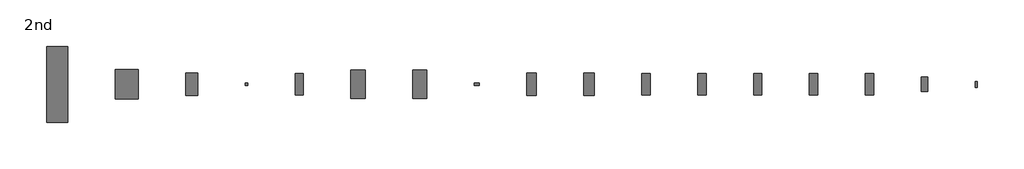
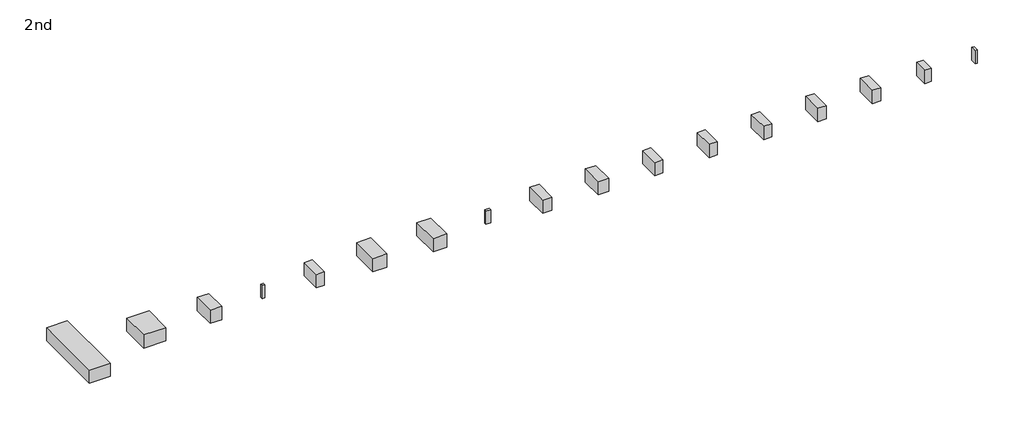
# One storey: 17 proxies.
"""IFC4 building model written with IfcOpenShell, lengths in millimetres."""

import ifcopenshell
import ifcopenshell.guid

model = None  # the IFC model being written
_history = None  # IfcOwnerHistory: only IFC2X3 demands one
_inside = {}  # id of a spatial element -> (the spatial element, [elements in it])
_under = {}  # id of a project, library or spatial element -> (it, [spatial elements below it])
_declared = {}  # id of a project -> (the project, [libraries it declares])
_typed = {}  # id of a type object -> (the type object, [elements of that type])
_made_of = {}  # id of a material, layer set ... -> (it, [elements and type objects made of it])


def new_model(schema):
    """Start an empty IFC model of exactly this schema.

    Asked for "IFC4X3", IfcOpenShell would pick the latest addendum, in which some entities
    have other attributes; the version numbers below select the first issue.
    IFC2X3 requires an IfcOwnerHistory on every rooted entity: one is made here for all.
    """
    global model, _history
    if schema == "IFC4X3":
        model = ifcopenshell.file(schema_version=(4, 3, 0, 0))
    else:
        model = ifcopenshell.file(schema=schema)
    _inside.clear()
    _under.clear()
    _declared.clear()
    _typed.clear()
    _made_of.clear()
    _history = None
    if model.schema == "IFC2X3":
        org = make("IfcOrganization", Name="unknown")
        user = make(
            "IfcPersonAndOrganization",
            ThePerson=make("IfcPerson", FamilyName="unknown"),
            TheOrganization=org,
        )
        app = make(
            "IfcApplication",
            ApplicationDeveloper=org,
            Version="unknown",
            ApplicationFullName="unknown",
            ApplicationIdentifier="unknown",
        )
        _history = make(
            "IfcOwnerHistory",
            OwningUser=user,
            OwningApplication=app,
            ChangeAction="ADDED",
            CreationDate=0,
        )
    return model


def make(cls, **values):
    """One entity of the class cls with the attributes given. An attribute that is None is left unset."""
    return model.create_entity(
        cls, **{name: value for name, value in values.items() if value is not None}
    )


def rooted(cls, **values):
    """An entity with a GlobalId (a new one), such as an element, a storey or a relation."""
    return make(cls, GlobalId=ifcopenshell.guid.new(), OwnerHistory=_history, **values)


def si_unit(unit_type, name, prefix=None):
    """IfcSIUnit, for example si_unit("LENGTHUNIT", "METRE", prefix="MILLI")."""
    return make("IfcSIUnit", UnitType=unit_type, Prefix=prefix, Name=name)


def assignment(units):
    """IfcUnitAssignment: the units of a project."""
    return None if units is None else make("IfcUnitAssignment", Units=units)


def point(xyz):
    """IfcCartesianPoint."""
    return None if xyz is None else make("IfcCartesianPoint", Coordinates=xyz)


def direction(xyz):
    """IfcDirection."""
    return None if xyz is None else make("IfcDirection", DirectionRatios=xyz)


def frame(location, z_axis=None, x_axis=None):
    """IfcAxis2Placement3D, a coordinate frame: its origin and axes. An axis left out is left unset."""
    return make(
        "IfcAxis2Placement3D",
        Location=point(location),
        Axis=direction(z_axis),
        RefDirection=direction(x_axis),
    )


def origin():
    """The frame at (0, 0, 0) with its axes left unset."""
    return frame((0.0, 0.0, 0.0))


def origin_with_axes():
    """The frame at (0, 0, 0) with the z axis (0, 0, 1) and the x axis (1, 0, 0) written out."""
    return frame((0.0, 0.0, 0.0), z_axis=(0.0, 0.0, 1.0), x_axis=(1.0, 0.0, 0.0))


def place(relative_to, where):
    """IfcLocalPlacement: puts the frame where relative to a parent placement (None: the world)."""
    return make(
        "IfcLocalPlacement", PlacementRelTo=relative_to, RelativePlacement=where
    )


def context(
    kind, dimensions, precision=None, world=None, true_north=None, identifier=None
):
    """IfcGeometricRepresentationContext, for example the 3D "Model" context."""
    return make(
        "IfcGeometricRepresentationContext",
        ContextIdentifier=identifier,
        ContextType=kind,
        CoordinateSpaceDimension=dimensions,
        Precision=precision,
        WorldCoordinateSystem=world,
        TrueNorth=true_north,
    )


def project(units=None, contexts=None):
    """IfcProject with its units and contexts."""
    return rooted(
        "IfcProject",
        Name="project",
        RepresentationContexts=contexts,
        UnitsInContext=assignment(units),
    )


def spatial(cls, under=None, at=None, **own):
    """A site, building, storey or space (cls), placed at a placement, below another one or the project."""
    s = rooted(cls, ObjectPlacement=at, **own)
    if under is not None:
        _under.setdefault(under.id(), (under, []))[1].append(s)
    return s


def polyline(points):
    """IfcPolyline through the points."""
    return make("IfcPolyline", Points=[point(p) for p in points])


def outline(outer, holes=None, kind="AREA"):
    """IfcArbitraryClosedProfileDef: a profile drawn as a closed curve; with holes, ...WithVoids."""
    if holes is None:
        return make("IfcArbitraryClosedProfileDef", ProfileType=kind, OuterCurve=outer)
    return make(
        "IfcArbitraryProfileDefWithVoids",
        ProfileType=kind,
        OuterCurve=outer,
        InnerCurves=holes,
    )


def extrude(swept, where, along, depth):
    """IfcExtrudedAreaSolid: the profile swept, set in the frame where, extruded along a direction by depth."""
    return make(
        "IfcExtrudedAreaSolid",
        SweptArea=swept,
        Position=where,
        ExtrudedDirection=direction(along),
        Depth=depth,
    )


def shape(context_of_items, identifier, shape_type, items):
    """IfcShapeRepresentation: the items that make up one representation, for example the "Body"."""
    return make(
        "IfcShapeRepresentation",
        ContextOfItems=context_of_items,
        RepresentationIdentifier=identifier,
        RepresentationType=shape_type,
        Items=items,
    )


def source(mapping_origin, context_of_items, identifier, shape_type, items):
    """IfcRepresentationMap: a shape defined once, which mapped items show again and again."""
    return make(
        "IfcRepresentationMap",
        MappingOrigin=mapping_origin,
        MappedRepresentation=shape(context_of_items, identifier, shape_type, items),
    )


def transform(
    local_origin,
    x_axis=None,
    y_axis=None,
    z_axis=None,
    scale=None,
    scale2=None,
    scale3=None,
    uniform=True,
):
    """IfcCartesianTransformationOperator3D, or its non-uniform kind. x_axis, y_axis, z_axis: its Axis1, 2, 3."""
    if uniform:
        return make(
            "IfcCartesianTransformationOperator3D",
            Axis1=direction(x_axis),
            Axis2=direction(y_axis),
            LocalOrigin=point(local_origin),
            Scale=scale,
            Axis3=direction(z_axis),
        )
    return make(
        "IfcCartesianTransformationOperator3DnonUniform",
        Axis1=direction(x_axis),
        Axis2=direction(y_axis),
        LocalOrigin=point(local_origin),
        Scale=scale,
        Axis3=direction(z_axis),
        Scale2=scale2,
        Scale3=scale3,
    )


def mapped(mapping_source, mapping_target):
    """IfcMappedItem: shows the shape of a source again, moved by a transform."""
    return make(
        "IfcMappedItem", MappingSource=mapping_source, MappingTarget=mapping_target
    )


def made_of(thing, what):
    """Note that an element or type object is made of a material, layer set ...; save() writes the relation."""
    if what is not None:
        _made_of.setdefault(what.id(), (what, []))[1].append(thing)
    return thing


def element(
    cls,
    number,
    at=None,
    inside=None,
    cuts=None,
    type_object=None,
    material=None,
    context=None,
    identifier="Body",
    shape_type=None,
    held_by="IfcProductDefinitionShape",
    body=None,
    shapes=None,
    **own,
):
    """One element of the class cls, such as IfcWall. Its Tag is "e" and its number.

    at: its placement. inside: the storey or other place that contains it. cuts: it is an
    opening in that element (IfcRelVoidsElement). A single representation is given by context,
    identifier, shape_type and body (its items); several are given by shapes. held_by: the class
    of the entity that holds the representations. save() writes the other relations.
    """
    e = rooted(cls, Tag="e%d" % number, ObjectPlacement=at, **own)
    if body is not None:
        shapes = [shape(context, identifier, shape_type, body)]
    if shapes is not None:
        e.Representation = make(held_by, Representations=shapes)
    if inside is not None:
        _inside.setdefault(inside.id(), (inside, []))[1].append(e)
    if cuts is not None:
        rooted(
            "IfcRelVoidsElement", RelatingBuildingElement=cuts, RelatedOpeningElement=e
        )
    if type_object is not None:
        _typed.setdefault(type_object.id(), (type_object, []))[1].append(e)
    return made_of(e, material)


def aggregate(whole, parts):
    """IfcRelAggregates: a whole, such as a stair, and the parts it consists of."""
    return rooted("IfcRelAggregates", RelatingObject=whole, RelatedObjects=parts)


def save(model, path):
    """Write the relations noted so far, then the file.

    IfcRelAggregates (storeys below a building ...), IfcRelContainedInSpatialStructure (elements
    in a storey), IfcRelDefinesByType, IfcRelAssociatesMaterial and IfcRelDeclares: one each for
    every whole, place, type object, material and project.
    """
    for whole, parts in _under.values():
        aggregate(whole, parts)
    for where, things in _inside.values():
        rooted(
            "IfcRelContainedInSpatialStructure",
            RelatedElements=things,
            RelatingStructure=where,
        )
    for kind, things in _typed.values():
        rooted("IfcRelDefinesByType", RelatedObjects=things, RelatingType=kind)
    for what, things in _made_of.values():
        rooted("IfcRelAssociatesMaterial", RelatedObjects=things, RelatingMaterial=what)
    for by, libraries in _declared.values():
        rooted("IfcRelDeclares", RelatingContext=by, RelatedDefinitions=libraries)
    model.write(path)


def generic_models_5634f436(model_context):
    return source(origin(), model_context, "Body", "SweptSolid", [
        extrude(outline(polyline([(1350.0, 3000.0), (1350.0, -3000.0), (-1350.0, -3000.0), (-1350.0, 3000.0), (1350.0, 3000.0)])), origin_with_axes(), (0.0, 0.0, 1.0), 6000.0),
    ])


def generic_models_71e2440f(model_context):
    return source(origin(), model_context, "Body", "SweptSolid", [
        extrude(outline(polyline([(500.0, 1250.0), (500.0, -1250.0), (-500.0, -1250.0), (-500.0, 1250.0), (500.0, 1250.0)])), origin_with_axes(), (0.0, 0.0, 1.0), 6000.0),
    ])


def generic_models_57c7875f(model_context):
    return source(origin(), model_context, "Body", "SweptSolid", [
        extrude(outline(polyline([(4500.0, 16000.0), (4500.0, -16000.0), (-4500.0, -16000.0), (-4500.0, 16000.0), (4500.0, 16000.0)])), origin_with_axes(), (0.0, 0.0, 1.0), 6000.0),
    ])


def generic_models_72d488a7(model_context):
    return source(origin(), model_context, "Body", "SweptSolid", [
        extrude(outline(polyline([(4800.0, 6250.0), (4800.0, -6250.0), (-4800.0, -6250.0), (-4800.0, 6250.0), (4800.0, 6250.0)])), origin_with_axes(), (0.0, 0.0, 1.0), 6000.0),
    ])


def generic_models_7902148a(model_context):
    return source(origin(), model_context, "Body", "SweptSolid", [
        extrude(outline(polyline([(2500.0, 4800.0), (2500.0, -4800.0), (-2500.0, -4800.0), (-2500.0, 4800.0), (2500.0, 4800.0)])), origin_with_axes(), (0.0, 0.0, 1.0), 6000.0),
    ])


def generic_models_ed4b717c(model_context):
    return source(origin(), model_context, "Body", "SweptSolid", [
        extrude(outline(polyline([(500.0, 500.0), (500.0, -500.0), (-500.0, -500.0), (-500.0, 500.0), (500.0, 500.0)])), origin_with_axes(), (0.0, 0.0, 1.0), 6000.0),
    ])


def generic_models_c01b8d6f(model_context):
    return source(origin(), model_context, "Body", "SweptSolid", [
        extrude(outline(polyline([(1750.0, 4500.0), (1750.0, -4500.0), (-1750.0, -4500.0), (-1750.0, 4500.0), (1750.0, 4500.0)])), origin_with_axes(), (0.0, 0.0, 1.0), 6000.0),
    ])


def generic_models_43059f4e(model_context):
    return source(origin(), model_context, "Body", "SweptSolid", [
        extrude(outline(polyline([(3000.0, 6000.0), (3000.0, -6000.0), (-3000.0, -6000.0), (-3000.0, 6000.0), (3000.0, 6000.0)])), origin_with_axes(), (0.0, 0.0, 1.0), 6000.0),
    ])


def generic_models_da00a96f(model_context):
    return source(origin(), model_context, "Body", "SweptSolid", [
        extrude(outline(polyline([(1000.0, 500.0), (1000.0, -500.0), (-1000.0, -500.0), (-1000.0, 500.0), (1000.0, 500.0)])), origin_with_axes(), (0.0, 0.0, 1.0), 6000.0),
    ])


def generic_models_3a820573(model_context):
    return source(origin(), model_context, "Body", "SweptSolid", [
        extrude(outline(polyline([(2000.0, 4750.0), (2000.0, -4750.0), (-2000.0, -4750.0), (-2000.0, 4750.0), (2000.0, 4750.0)])), origin_with_axes(), (0.0, 0.0, 1.0), 6000.0),
    ])


def generic_models_96097b63(model_context):
    return source(origin(), model_context, "Body", "SweptSolid", [
        extrude(outline(polyline([(2250.0, 4800.0), (2250.0, -4800.0), (-2250.0, -4800.0), (-2250.0, 4800.0), (2250.0, 4800.0)])), origin_with_axes(), (0.0, 0.0, 1.0), 6000.0),
    ])


model = new_model("IFC4")

# Units and contexts
model_context = context("Model", 3, world=origin())
ifc_project = project(units=[si_unit("LENGTHUNIT", "METRE", prefix="MILLI")], contexts=[model_context])

# Site, building, storey
site = spatial("IfcSite", under=ifc_project)
building = spatial("IfcBuilding", under=site)
storey = spatial("IfcBuildingStorey", under=building, Name="2nd", Elevation=14000.0)

# Proxies
placement = place(None, origin())
generic_models_shape = generic_models_5634f436(model_context)
element("IfcBuildingElementProxy", 1, Name="Space Planning Box_hec : Space Planning Box_hec", ObjectType="Space Planning Box_hec : Space Planning Box_hec", at=placement, inside=storey, context=model_context, shape_type="MappedRepresentation", body=[
    mapped(generic_models_shape, transform((369450.0, 168000.0, 14000.0), x_axis=(1.0, 0.0, 0.0), y_axis=(0.0, 1.0, 0.0), z_axis=(0.0, 0.0, 1.0))),
])
generic_models_2_shape = generic_models_71e2440f(model_context)
element("IfcBuildingElementProxy", 2, Name="Space Planning Box_hec : Space Planning Box_hec", ObjectType="Space Planning Box_hec : Space Planning Box_hec", at=placement, inside=storey, context=model_context, shape_type="MappedRepresentation", body=[
    mapped(generic_models_2_shape, transform((391300.0, 168000.0, 14000.0), x_axis=(1.0, 0.0, 0.0), y_axis=(0.0, 1.0, 0.0), z_axis=(0.0, 0.0, 1.0))),
])
generic_models_3_shape = generic_models_57c7875f(model_context)
element("IfcBuildingElementProxy", 3, Name="Space Planning Box_hec : Space Planning Box_hec", ObjectType="Space Planning Box_hec : Space Planning Box_hec", at=placement, inside=storey, context=model_context, shape_type="MappedRepresentation", body=[
    mapped(generic_models_3_shape, transform((4500.0, 168000.0, 14000.0), x_axis=(1.0, 0.0, 0.0), y_axis=(0.0, 1.0, 0.0), z_axis=(0.0, 0.0, 1.0))),
])
generic_models_4_shape = generic_models_72d488a7(model_context)
element("IfcBuildingElementProxy", 4, Name="Space Planning Box_hec : Space Planning Box_hec", ObjectType="Space Planning Box_hec : Space Planning Box_hec", at=placement, inside=storey, context=model_context, shape_type="MappedRepresentation", body=[
    mapped(generic_models_4_shape, transform((33800.0, 168000.0, 14000.0), x_axis=(1.0, 0.0, 0.0), y_axis=(0.0, 1.0, 0.0), z_axis=(0.0, 0.0, 1.0))),
])
generic_models_5_shape = generic_models_7902148a(model_context)
element("IfcBuildingElementProxy", 5, Name="Space Planning Box_hec : Space Planning Box_hec", ObjectType="Space Planning Box_hec : Space Planning Box_hec", at=placement, inside=storey, context=model_context, shape_type="MappedRepresentation", body=[
    mapped(generic_models_5_shape, transform((61100.0, 168000.0, 14000.0), x_axis=(1.0, 0.0, 0.0), y_axis=(0.0, 1.0, 0.0), z_axis=(0.0, 0.0, 1.0))),
])
generic_models_6_shape = generic_models_ed4b717c(model_context)
element("IfcBuildingElementProxy", 6, Name="Space Planning Box_hec : Space Planning Box_hec", ObjectType="Space Planning Box_hec : Space Planning Box_hec", at=placement, inside=storey, context=model_context, shape_type="MappedRepresentation", body=[
    mapped(generic_models_6_shape, transform((84100.0, 168000.0, 14000.0), x_axis=(1.0, 0.0, 0.0), y_axis=(0.0, 1.0, 0.0), z_axis=(0.0, 0.0, 1.0))),
])
generic_models_7_shape = generic_models_c01b8d6f(model_context)
element("IfcBuildingElementProxy", 7, Name="Space Planning Box_hec : Space Planning Box_hec", ObjectType="Space Planning Box_hec : Space Planning Box_hec", at=placement, inside=storey, context=model_context, shape_type="MappedRepresentation", body=[
    mapped(generic_models_7_shape, transform((106350.0, 168000.0, 14000.0), x_axis=(1.0, 0.0, 0.0), y_axis=(0.0, 1.0, 0.0), z_axis=(0.0, 0.0, 1.0))),
])
element("IfcBuildingElementProxy", 8, Name="Space Planning Box_hec : Space Planning Box_hec", ObjectType="Space Planning Box_hec : Space Planning Box_hec", at=placement, inside=storey, context=model_context, shape_type="MappedRepresentation", body=[
    mapped(generic_models_7_shape, transform((252350.0, 168000.0, 14000.0), x_axis=(1.0, 0.0, 0.0), y_axis=(0.0, 1.0, 0.0), z_axis=(0.0, 0.0, 1.0))),
])
element("IfcBuildingElementProxy", 9, Name="Space Planning Box_hec : Space Planning Box_hec", ObjectType="Space Planning Box_hec : Space Planning Box_hec", at=placement, inside=storey, context=model_context, shape_type="MappedRepresentation", body=[
    mapped(generic_models_7_shape, transform((275850.0, 168000.0, 14000.0), x_axis=(1.0, 0.0, 0.0), y_axis=(0.0, 1.0, 0.0), z_axis=(0.0, 0.0, 1.0))),
])
element("IfcBuildingElementProxy", 10, Name="Space Planning Box_hec : Space Planning Box_hec", ObjectType="Space Planning Box_hec : Space Planning Box_hec", at=placement, inside=storey, context=model_context, shape_type="MappedRepresentation", body=[
    mapped(generic_models_7_shape, transform((299350.0, 168000.0, 14000.0), x_axis=(1.0, 0.0, 0.0), y_axis=(0.0, 1.0, 0.0), z_axis=(0.0, 0.0, 1.0))),
])
element("IfcBuildingElementProxy", 11, Name="Space Planning Box_hec : Space Planning Box_hec", ObjectType="Space Planning Box_hec : Space Planning Box_hec", at=placement, inside=storey, context=model_context, shape_type="MappedRepresentation", body=[
    mapped(generic_models_7_shape, transform((322850.0, 168000.0, 14000.0), x_axis=(1.0, 0.0, 0.0), y_axis=(0.0, 1.0, 0.0), z_axis=(0.0, 0.0, 1.0))),
])
element("IfcBuildingElementProxy", 12, Name="Space Planning Box_hec : Space Planning Box_hec", ObjectType="Space Planning Box_hec : Space Planning Box_hec", at=placement, inside=storey, context=model_context, shape_type="MappedRepresentation", body=[
    mapped(generic_models_7_shape, transform((346350.0, 168000.0, 14000.0), x_axis=(1.0, 0.0, 0.0), y_axis=(0.0, 1.0, 0.0), z_axis=(0.0, 0.0, 1.0))),
])
generic_models_8_shape = generic_models_43059f4e(model_context)
element("IfcBuildingElementProxy", 13, Name="Space Planning Box_hec : Space Planning Box_hec", ObjectType="Space Planning Box_hec : Space Planning Box_hec", at=placement, inside=storey, context=model_context, shape_type="MappedRepresentation", body=[
    mapped(generic_models_8_shape, transform((131100.0, 168000.0, 14000.0), x_axis=(1.0, 0.0, 0.0), y_axis=(0.0, 1.0, 0.0), z_axis=(0.0, 0.0, 1.0))),
])
element("IfcBuildingElementProxy", 14, Name="Space Planning Box_hec : Space Planning Box_hec", ObjectType="Space Planning Box_hec : Space Planning Box_hec", at=placement, inside=storey, context=model_context, shape_type="MappedRepresentation", body=[
    mapped(generic_models_8_shape, transform((157100.0, 168000.0, 14000.0), x_axis=(1.0, 0.0, 0.0), y_axis=(0.0, 1.0, 0.0), z_axis=(0.0, 0.0, 1.0))),
])
generic_models_9_shape = generic_models_da00a96f(model_context)
element("IfcBuildingElementProxy", 15, Name="Space Planning Box_hec : Space Planning Box_hec", ObjectType="Space Planning Box_hec : Space Planning Box_hec", at=placement, inside=storey, context=model_context, shape_type="MappedRepresentation", body=[
    mapped(generic_models_9_shape, transform((181100.0, 168000.0, 14000.0), x_axis=(1.0, 0.0, 0.0), y_axis=(0.0, 1.0, 0.0), z_axis=(0.0, 0.0, 1.0))),
])
generic_models_10_shape = generic_models_3a820573(model_context)
element("IfcBuildingElementProxy", 16, Name="Space Planning Box_hec : Space Planning Box_hec", ObjectType="Space Planning Box_hec : Space Planning Box_hec", at=placement, inside=storey, context=model_context, shape_type="MappedRepresentation", body=[
    mapped(generic_models_10_shape, transform((204100.0, 168000.0, 14000.0), x_axis=(1.0, 0.0, 0.0), y_axis=(0.0, 1.0, 0.0), z_axis=(0.0, 0.0, 1.0))),
])
generic_models_11_shape = generic_models_96097b63(model_context)
element("IfcBuildingElementProxy", 17, Name="Space Planning Box_hec : Space Planning Box_hec", ObjectType="Space Planning Box_hec : Space Planning Box_hec", at=placement, inside=storey, context=model_context, shape_type="MappedRepresentation", body=[
    mapped(generic_models_11_shape, transform((228350.0, 168000.0, 14000.0), x_axis=(1.0, 0.0, 0.0), y_axis=(0.0, 1.0, 0.0), z_axis=(0.0, 0.0, 1.0))),
])

save(model, "model.ifc")

# Revit data of these elements
# Project information
#   Project Issue Date = "Issue Date"
#   Project Status = "Project Status"
#   Client Name = "Owner"
#   Project Address = "Enter address here"
#   Project Name = "Project Name"
#   Project Number = "Project Number"
# Type "Space Planning Box_hec : Space Planning Box_hec"
#   Type Comments = "..."
#   Room Name [instance default] = "?"
#   Interior Finish [instance default] = ""
#   Exterior Finish [instance default] = ""
#   Department [instance default] = ""
#   Assembly Code = "..."
#   Width [instance default] = 1524 mm
#   Program Area [instance default] = 0 m²
#   Length [instance default] = 1524 mm
#   Height [instance default] = 1524 mm
#   Area [instance default] = 2.32258 m²
#   Fill Color [instance default] = Cyan
#   Default Elevation = 0
# Element 1 (IfcBuildingElementProxy, "Space Planning Box_hec : Space Planning Box_hec")
#   Room Name = "Duct Shaft"
#   Interior Finish = "NA"
#   Exterior Finish = "EF1"
#   Department = "HV"
#   Width = 2700 mm
#   Program Area = 16.2 m²
#   Length = 6000 mm
#   Height = 6000 mm
#   Area = 16.2 m²
#   Fill Color = Pink
#   Phase Created = New Construction
#   Materials on its faces: "Pink"
# Element 2 (IfcBuildingElementProxy, "Space Planning Box_hec : Space Planning Box_hec")
#   Room Name = "Pipe Shaft"
#   Interior Finish = "NA"
#   Exterior Finish = "EF1"
#   Department = "HV"
#   Width = 1000 mm
#   Program Area = 2.5 m²
#   Length = 2500 mm
#   Height = 6000 mm
#   Area = 2.5 m²
#   Fill Color = Pink
#   Phase Created = New Construction
#   Materials on its faces: "Pink"
# Element 3 (IfcBuildingElementProxy, "Space Planning Box_hec : Space Planning Box_hec")
#   Room Name = "Central Control Room"
#   Interior Finish = "IF3"
#   Exterior Finish = "EF1"
#   Department = "CI"
#   Width = 9000 mm
#   Program Area = 288 m²
#   Length = 32000 mm
#   Height = 6000 mm
#   Area = 288 m²
#   Fill Color = Lime
#   Phase Created = New Construction
#   Materials on its faces: "Lime"
# Element 4 (IfcBuildingElementProxy, "Space Planning Box_hec : Space Planning Box_hec")
#   Room Name = "Engineer Room"
#   Interior Finish = "IF3"
#   Exterior Finish = "EF1"
#   Department = "CI"
#   Width = 9600 mm
#   Program Area = 120 m²
#   Length = 12500 mm
#   Height = 6000 mm
#   Area = 120 m²
#   Fill Color = Lime
#   Phase Created = New Construction
#   Materials on its faces: "Lime"
# Element 5 (IfcBuildingElementProxy, "Space Planning Box_hec : Space Planning Box_hec")
#   Room Name = "Document Room"
#   Interior Finish = "IF2-1"
#   Exterior Finish = "EF1"
#   Department = "AR"
#   Width = 5000 mm
#   Program Area = 48 m²
#   Length = 9600 mm
#   Height = 6000 mm
#   Area = 48 m²
#   Fill Color = Lavender
#   Phase Created = New Construction
#   Materials on its faces: "Lavender"
# Element 6 (IfcBuildingElementProxy, "Space Planning Box_hec : Space Planning Box_hec")
#   Room Name = "Fire Gas Room"
#   Interior Finish = "IF1"
#   Exterior Finish = "EF1"
#   Department = "SF"
#   Width = 1000 mm
#   Program Area = 0 m²
#   Length = 1000 mm
#   Height = 6000 mm
#   Area = 1 m²
#   Fill Color = Cyan
#   Phase Created = New Construction
#   Materials on its faces: "Cyan"
# Element 7 (IfcBuildingElementProxy, "Space Planning Box_hec : Space Planning Box_hec")
#   Room Name = "Kitch & Lunch Room"
#   Interior Finish = "IF2-1"
#   Exterior Finish = "EF1"
#   Department = "AR"
#   Width = 3500 mm
#   Program Area = 31.5 m²
#   Length = 9000 mm
#   Height = 6000 mm
#   Area = 31.5 m²
#   Fill Color = Lavender
#   Phase Created = New Construction
#   Materials on its faces: "Lavender"
# Element 8 (IfcBuildingElementProxy, "Space Planning Box_hec : Space Planning Box_hec")
#   Room Name = "LOTO Office Room"
#   Interior Finish = "IF2-1"
#   Exterior Finish = "EF1"
#   Department = "AR"
#   Width = 3500 mm
#   Program Area = 31.5 m²
#   Length = 9000 mm
#   Height = 6000 mm
#   Area = 31.5 m²
#   Fill Color = Lavender
#   Phase Created = New Construction
#   Materials on its faces: "Lavender"
# Element 9 (IfcBuildingElementProxy, "Space Planning Box_hec : Space Planning Box_hec")
#   Room Name = "Shower Room (F)"
#   Interior Finish = "IF5"
#   Exterior Finish = "EF1"
#   Department = "AR"
#   Width = 3500 mm
#   Program Area = 31.5 m²
#   Length = 9000 mm
#   Height = 6000 mm
#   Area = 31.5 m²
#   Fill Color = Lavender
#   Phase Created = New Construction
#   Materials on its faces: "Lavender"
# Element 10 (IfcBuildingElementProxy, "Space Planning Box_hec : Space Planning Box_hec")
#   Room Name = "Locker Room (F)"
#   Interior Finish = "IF2-1"
#   Exterior Finish = "EF1"
#   Department = "AR"
#   Width = 3500 mm
#   Program Area = 31.5 m²
#   Length = 9000 mm
#   Height = 6000 mm
#   Area = 31.5 m²
#   Fill Color = Lavender
#   Phase Created = New Construction
#   Materials on its faces: "Lavender"
# Element 11 (IfcBuildingElementProxy, "Space Planning Box_hec : Space Planning Box_hec")
#   Room Name = "Shower Room (M)"
#   Interior Finish = "IF5"
#   Exterior Finish = "EF1"
#   Department = "AR"
#   Width = 3500 mm
#   Program Area = 31.5 m²
#   Length = 9000 mm
#   Height = 6000 mm
#   Area = 31.5 m²
#   Fill Color = Lavender
#   Phase Created = New Construction
#   Materials on its faces: "Lavender"
# Element 12 (IfcBuildingElementProxy, "Space Planning Box_hec : Space Planning Box_hec")
#   Room Name = "Locker Room (M)"
#   Interior Finish = "IF2-1"
#   Exterior Finish = "EF1"
#   Department = "AR"
#   Width = 3500 mm
#   Program Area = 31.5 m²
#   Length = 9000 mm
#   Height = 6000 mm
#   Area = 31.5 m²
#   Fill Color = Lavender
#   Phase Created = New Construction
#   Materials on its faces: "Lavender"
# Element 13 (IfcBuildingElementProxy, "Space Planning Box_hec : Space Planning Box_hec")
#   Room Name = "Toilet (M)"
#   Interior Finish = "IF5"
#   Exterior Finish = "EF1"
#   Department = "AR"
#   Width = 6000 mm
#   Program Area = 72 m²
#   Length = 12000 mm
#   Height = 6000 mm
#   Area = 72 m²
#   Fill Color = Lavender
#   Phase Created = New Construction
#   Materials on its faces: "Lavender"
# Element 14 (IfcBuildingElementProxy, "Space Planning Box_hec : Space Planning Box_hec")
#   Room Name = "Toilet (F)"
#   Interior Finish = "IF5"
#   Exterior Finish = "EF1"
#   Department = "AR"
#   Width = 6000 mm
#   Program Area = 72 m²
#   Length = 12000 mm
#   Height = 6000 mm
#   Area = 72 m²
#   Fill Color = Lavender
#   Phase Created = New Construction
#   Materials on its faces: "Lavender"
# Element 15 (IfcBuildingElementProxy, "Space Planning Box_hec : Space Planning Box_hec")
#   Room Name = "Corridor"
#   Interior Finish = "IF2-1"
#   Exterior Finish = "EF1"
#   Department = "AR"
#   Width = 2000 mm
#   Program Area = 0 m²
#   Length = 1000 mm
#   Height = 6000 mm
#   Area = 2 m²
#   Fill Color = Lavender
#   Phase Created = New Construction
#   Materials on its faces: "Lavender"
# Element 16 (IfcBuildingElementProxy, "Space Planning Box_hec : Space Planning Box_hec")
#   Room Name = "Stairway"
#   Interior Finish = "IF2"
#   Exterior Finish = "EF1"
#   Department = "AR"
#   Width = 4000 mm
#   Program Area = 38 m²
#   Length = 9500 mm
#   Height = 6000 mm
#   Area = 38 m²
#   Fill Color = Lavender
#   Phase Created = New Construction
#   Materials on its faces: "Lavender"
# Element 17 (IfcBuildingElementProxy, "Space Planning Box_hec : Space Planning Box_hec")
#   Room Name = "Shift Office Room"
#   Interior Finish = "IF2-1"
#   Exterior Finish = "EF1"
#   Department = "AR"
#   Width = 4500 mm
#   Program Area = 43.2 m²
#   Length = 9600 mm
#   Height = 6000 mm
#   Area = 43.2 m²
#   Fill Color = Lavender
#   Phase Created = New Construction
#   Materials on its faces: "Lavender"
# Materials
#   "Cyan": class "Generic", colour RGB 0 255 255, transparency 0.2, Cost = 0
#   "Pink": class "Generic", colour RGB 255 105 180, transparency 0.2, Cost = 0
#   "Lime": class "Generic", colour RGB 0 255 0, transparency 0.2, Cost = 0
#   "Lavender": class "Generic", colour RGB 186 85 211, transparency 0.2, Cost = 0
